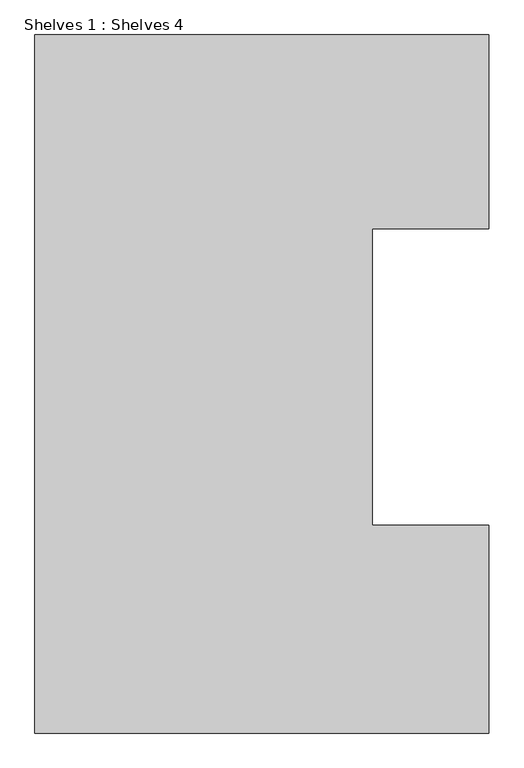
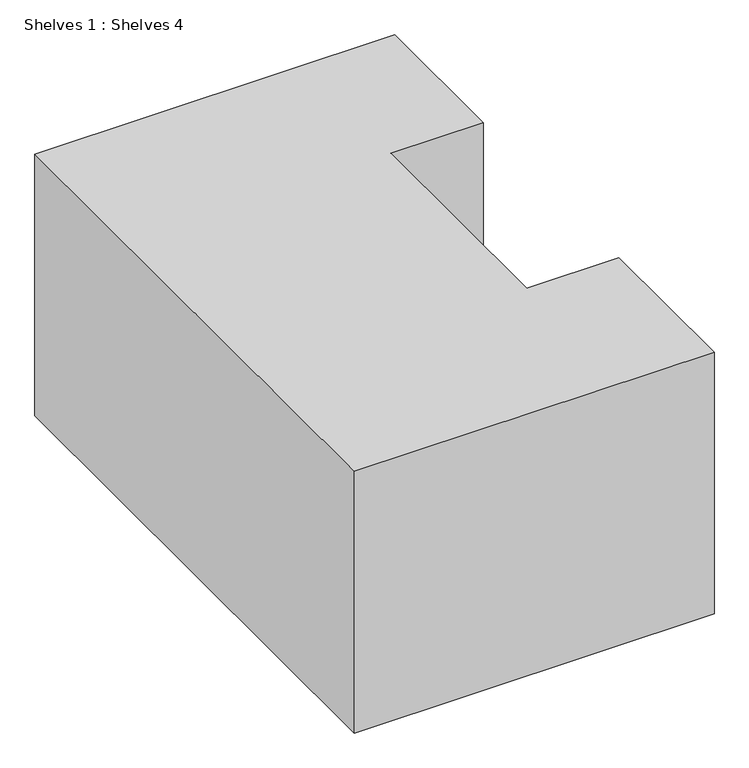
"""IFC4 building model written with IfcOpenShell, lengths in millimetres: furniture geometry, Shelves 1 : Shelves 4."""

from ifc_helpers import new_model, si_unit, origin, origin_with_axes, place, context, project, spatial, polyline, outline, extrude, source, transform, mapped, element, save


def shelves_1_shelves_4_b6e6bccd(model_context):
    return source(origin(), model_context, "Body", "SweptSolid", [
        extrude(outline(polyline([(15968.4036204, 8606.3270218), (17949.6036204, 8606.3270218), (17949.6036204, 7760.9615366), (17441.6036204, 7760.9615366), (17441.6036204, 6465.5615366), (17949.6036204, 6465.5615366), (17949.6036204, 5558.3270218), (15968.4036204, 5558.3270218), (15968.4036204, 8606.3270218)])), origin_with_axes(), (0.0, 0.0, 1.0), 1524.0),
    ])


if __name__ == "__main__":
    model = new_model("IFC4")
    model_context = context("Model", 3, world=origin())
    ifc_project = project(units=[si_unit("LENGTHUNIT", "METRE", prefix="MILLI")], contexts=[model_context])
    site = spatial("IfcSite", under=ifc_project)
    building = spatial("IfcBuilding", under=site)
    placement = place(None, origin())
    shelves_1_shelves_4_shape = shelves_1_shelves_4_b6e6bccd(model_context)
    element("IfcFurniture", 1, ObjectType="Shelves 1 : Shelves 4", at=placement, inside=building, context=model_context, shape_type="MappedRepresentation", body=[
        mapped(shelves_1_shelves_4_shape, transform((0.0, 0.0, 0.0), x_axis=(1.0, 0.0, 0.0), y_axis=(0.0, 1.0, 0.0), z_axis=(0.0, 0.0, 1.0))),
    ])
    save(model, "model.ifc")
